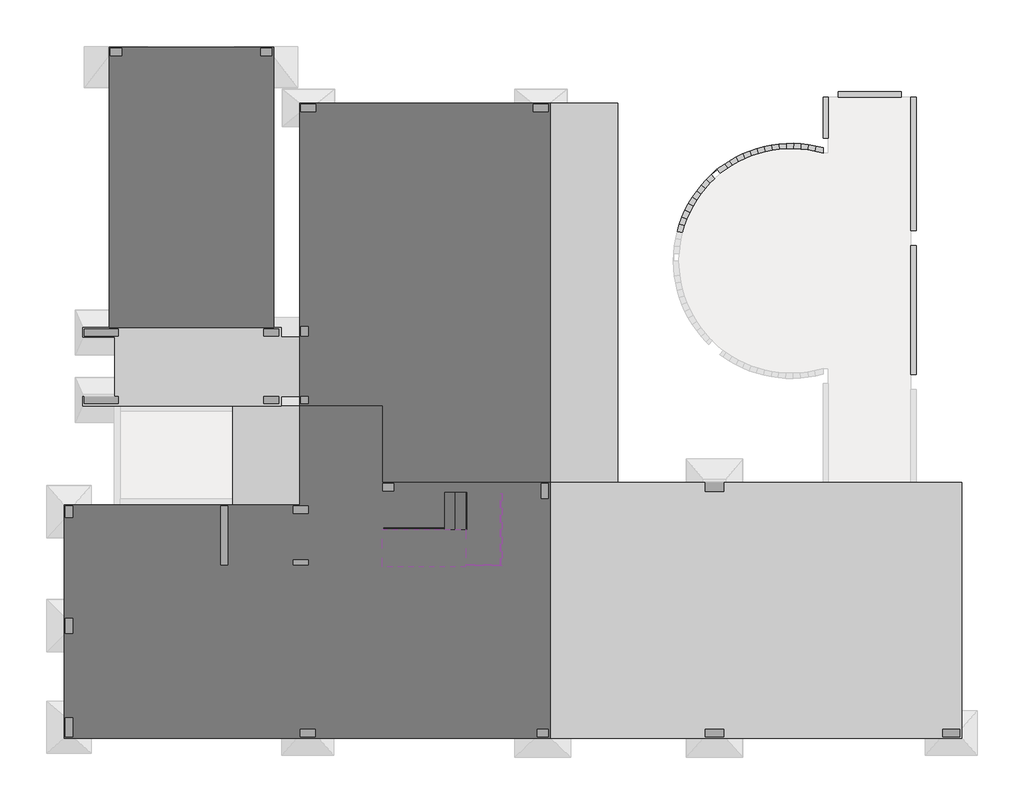
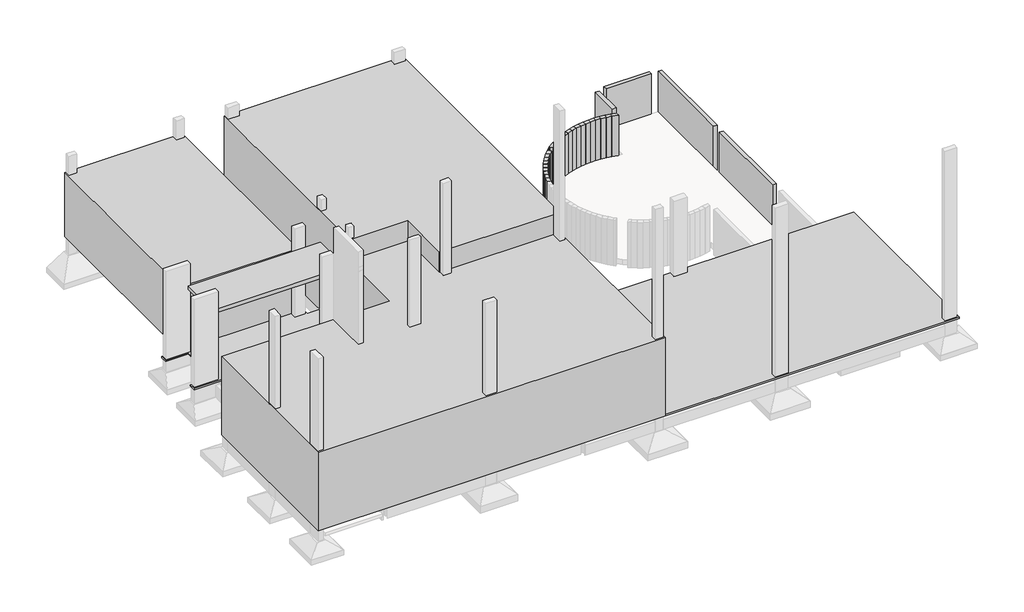
# One storey, part 4 of 4: 27 beams, 7 proxies, 6 railings, 2 stair flights, 1 slab.
# Revit data of these elements (continued)
# Element 2 (IfcBeam, "TQS - Viga retangular : 14.0 x 180.0") (continued)
#   Titulo = "VP6"
#   Chave = "-1017"
#   Tipo Elemento = "Viga"
#   SHA1 = "22C0BDACD46D49F6E4190D80621E2138C68CD36C"
#   Revisão = ""
#   Tipo de carga = ""
#   Divisor de flexao = ""
#   Secao = ""
#   Configuracao = ""
#   Angulo (graus) = ""
#   Detalhamento = ""
#   Casos de vento manual = ""
#   Tipo = ""
#   Alcas = ""
#   Furos = ""
#   Pino = ""
#   Distribuicao = ""
#   Solidarizado = ""
#   Solidarizar na montagem = ""
#   Unir com o próximo = ""
#   Grupo pre moldado = ""
#   Verificado = ""
#   Concreto C = ""
#   Taxa de armadura (kgf/m³) = 0
#   Carga (tf/m²) = 0
#   Carga (tf/m) = 0
#   Carga (tf) = 0
#   Altura = 1.80 m
#   Rebaixo = 0.15 m
#   Largura = 0.14 m
#   Distancia a face = 0.00 m
#   Distancia ao eixo = 0.00 m
#   Altura gerber esquerda = 0.00 m
#   Largura gerber esquerda = 0.00 m
#   Altura gerber direita = 0.00 m
#   Largura gerber direita = 0.00 m
#   Resultado de Ensaios fck (MPa) = 0
#   Unique TQS ID = -1017
#   Principal = yes
#   Structural Material = none
#   Phase Created = CC_AP/ESTR
# Element 3 (IfcBeam, "TQS - Viga retangular : 14.0 x 180.0")
#   Uso = "ESTRUTURA"
#   Titulo = "VP6"
#   Chave = "-1018"
#   Tipo Elemento = "Viga"
#   SHA1 = "D04A2C827C3C8BC1853343DA7F217DB9B9B2F05D"
#   Revisão = ""
#   Tipo de carga = ""
#   Divisor de flexao = ""
#   Secao = ""
#   Configuracao = ""
#   Angulo (graus) = ""
#   Detalhamento = ""
#   Casos de vento manual = ""
#   Tipo = ""
#   Alcas = ""
#   Furos = ""
#   Pino = ""
#   Distribuicao = ""
#   Solidarizado = ""
#   Solidarizar na montagem = ""
#   Unir com o próximo = ""
#   Grupo pre moldado = ""
#   Verificado = ""
#   Concreto C = ""
#   Taxa de armadura (kgf/m³) = 0
#   Carga (tf/m²) = 0
#   Carga (tf/m) = 0
#   Carga (tf) = 0
#   Altura = 1.80 m
#   Rebaixo = 0.15 m
#   Largura = 0.14 m
#   Distancia a face = 0.00 m
#   Distancia ao eixo = 0.00 m
#   Altura gerber esquerda = 0.00 m
#   Largura gerber esquerda = 0.00 m
#   Altura gerber direita = 0.00 m
#   Largura gerber direita = 0.00 m
#   Resultado de Ensaios fck (MPa) = 0
#   Unique TQS ID = -1018
#   Principal = yes
#   Structural Material = none
#   Phase Created = CC_AP/ESTR
# Element 4 (IfcBeam, "TQS - Viga retangular : 14.0 x 180.0")
#   Uso = "ESTRUTURA"
#   Titulo = "VP6"
#   Chave = "-1019"
#   Tipo Elemento = "Viga"
#   SHA1 = "0D182E2612785E293A5A4969EBA47990CD3E9117"
#   Revisão = ""
#   Tipo de carga = ""
#   Divisor de flexao = ""
#   Secao = ""
#   Configuracao = ""
#   Angulo (graus) = ""
#   Detalhamento = ""
#   Casos de vento manual = ""
#   Tipo = ""
#   Alcas = ""
#   Furos = ""
#   Pino = ""
#   Distribuicao = ""
#   Solidarizado = ""
#   Solidarizar na montagem = ""
#   Unir com o próximo = ""
#   Grupo pre moldado = ""
#   Verificado = ""
#   Concreto C = ""
#   Taxa de armadura (kgf/m³) = 0
#   Carga (tf/m²) = 0
#   Carga (tf/m) = 0
#   Carga (tf) = 0
#   Altura = 1.80 m
#   Rebaixo = 0.15 m
#   Largura = 0.14 m
#   Distancia a face = 0.00 m
#   Distancia ao eixo = 0.00 m
#   Altura gerber esquerda = 0.00 m
#   Largura gerber esquerda = 0.00 m
#   Altura gerber direita = 0.00 m
#   Largura gerber direita = 0.00 m
#   Resultado de Ensaios fck (MPa) = 0
#   Unique TQS ID = -1019
#   Principal = yes
#   Structural Material = none
#   Phase Created = CC_AP/ESTR
# Element 5 (IfcBeam, "TQS - Viga retangular : 14.0 x 180.0")
#   Uso = "ESTRUTURA"
#   Titulo = "VP6"
#   Chave = "-1020"
#   Tipo Elemento = "Viga"
#   SHA1 = "8A5DF36B72EBE22F2A453D6F9BADDE3EA3E2A9B4"
#   Revisão = ""
#   Tipo de carga = ""
#   Divisor de flexao = ""
#   Secao = ""
#   Configuracao = ""
#   Angulo (graus) = ""
#   Detalhamento = ""
#   Casos de vento manual = ""
#   Tipo = ""
#   Alcas = ""
#   Furos = ""
#   Pino = ""
#   Distribuicao = ""
#   Solidarizado = ""
#   Solidarizar na montagem = ""
#   Unir com o próximo = ""
#   Grupo pre moldado = ""
#   Verificado = ""
#   Concreto C = ""
#   Taxa de armadura (kgf/m³) = 0
#   Carga (tf/m²) = 0
#   Carga (tf/m) = 0
#   Carga (tf) = 0
#   Altura = 1.80 m
#   Rebaixo = 0.15 m
#   Largura = 0.14 m
#   Distancia a face = 0.00 m
#   Distancia ao eixo = 0.00 m
#   Altura gerber esquerda = 0.00 m
#   Largura gerber esquerda = 0.00 m
#   Altura gerber direita = 0.00 m
#   Largura gerber direita = 0.00 m
#   Resultado de Ensaios fck (MPa) = 0
#   Unique TQS ID = -1020
#   Principal = yes
#   Structural Material = none
#   Phase Created = CC_AP/ESTR
# Element 6 (IfcBeam, "TQS - Viga retangular : 14.0 x 180.0")
#   Uso = "ESTRUTURA"
#   Titulo = "VP6"
#   Chave = "-1021"
#   Tipo Elemento = "Viga"
#   SHA1 = "E996D88AC41B572457E87FBE2BFAA83C91B590B4"
#   Revisão = ""
#   Tipo de carga = ""
#   Divisor de flexao = ""
#   Secao = ""
#   Configuracao = ""
#   Angulo (graus) = ""
#   Detalhamento = ""
#   Casos de vento manual = ""
#   Tipo = ""
#   Alcas = ""
#   Furos = ""
#   Pino = ""
#   Distribuicao = ""
#   Solidarizado = ""
#   Solidarizar na montagem = ""
#   Unir com o próximo = ""
#   Grupo pre moldado = ""
#   Verificado = ""
#   Concreto C = ""
#   Taxa de armadura (kgf/m³) = 0
#   Carga (tf/m²) = 0
#   Carga (tf/m) = 0
#   Carga (tf) = 0
#   Altura = 1.80 m
#   Rebaixo = 0.15 m
#   Largura = 0.14 m
#   Distancia a face = 0.00 m
#   Distancia ao eixo = 0.00 m
#   Altura gerber esquerda = 0.00 m
#   Largura gerber esquerda = 0.00 m
#   Altura gerber direita = 0.00 m
#   Largura gerber direita = 0.00 m
#   Resultado de Ensaios fck (MPa) = 0
#   Unique TQS ID = -1021
#   Principal = yes
#   Structural Material = none
#   Phase Created = CC_AP/ESTR
# Element 7 (IfcBeam, "TQS - Viga retangular : 14.0 x 180.0")
#   Uso = "ESTRUTURA"
#   Titulo = "VP6"
#   Chave = "-1022"
#   Tipo Elemento = "Viga"
#   SHA1 = "0B33ED0C5CE953F65B7DD0F51C60662F46F82846"
#   Revisão = ""
#   Tipo de carga = ""
#   Divisor de flexao = ""
#   Secao = ""
#   Configuracao = ""
#   Angulo (graus) = ""
#   Detalhamento = ""
#   Casos de vento manual = ""
#   Tipo = ""
#   Alcas = ""
#   Furos = ""
#   Pino = ""
#   Distribuicao = ""
#   Solidarizado = ""
#   Solidarizar na montagem = ""
#   Unir com o próximo = ""
#   Grupo pre moldado = ""
#   Verificado = ""
#   Concreto C = ""
#   Taxa de armadura (kgf/m³) = 0
#   Carga (tf/m²) = 0
#   Carga (tf/m) = 0
#   Carga (tf) = 0
#   Altura = 1.80 m
#   Rebaixo = 0.15 m
#   Largura = 0.14 m
#   Distancia a face = 0.00 m
#   Distancia ao eixo = 0.00 m
#   Altura gerber esquerda = 0.00 m
#   Largura gerber esquerda = 0.00 m
#   Altura gerber direita = 0.00 m
#   Largura gerber direita = 0.00 m
#   Resultado de Ensaios fck (MPa) = 0
#   Unique TQS ID = -1022
#   Principal = yes
#   Structural Material = none
#   Phase Created = CC_AP/ESTR
# Element 8 (IfcBeam, "TQS - Viga retangular : 14.0 x 180.0")
#   Uso = "ESTRUTURA"
#   Titulo = "VP6"
#   Chave = "-1023"
#   Tipo Elemento = "Viga"
#   SHA1 = "7A0208B774D9472BDEB9F4D9C600465610707295"
#   Revisão = ""
#   Tipo de carga = ""
#   Divisor de flexao = ""
#   Secao = ""
#   Configuracao = ""
#   Angulo (graus) = ""
#   Detalhamento = ""
#   Casos de vento manual = ""
#   Tipo = ""
#   Alcas = ""
#   Furos = ""
#   Pino = ""
#   Distribuicao = ""
#   Solidarizado = ""
#   Solidarizar na montagem = ""
#   Unir com o próximo = ""
#   Grupo pre moldado = ""
#   Verificado = ""
#   Concreto C = ""
#   Taxa de armadura (kgf/m³) = 0
#   Carga (tf/m²) = 0
#   Carga (tf/m) = 0
#   Carga (tf) = 0
#   Altura = 1.80 m
#   Rebaixo = 0.15 m
#   Largura = 0.14 m
#   Distancia a face = 0.00 m
#   Distancia ao eixo = 0.00 m
#   Altura gerber esquerda = 0.00 m
#   Largura gerber esquerda = 0.00 m
#   Altura gerber direita = 0.00 m
#   Largura gerber direita = 0.00 m
#   Resultado de Ensaios fck (MPa) = 0
#   Unique TQS ID = -1023
#   Principal = yes
#   Structural Material = none
#   Phase Created = CC_AP/ESTR
# Element 9 (IfcBeam, "TQS - Viga retangular : 14.0 x 180.0")
#   Uso = "ESTRUTURA"
#   Titulo = "VP6"
#   Chave = "-1024"
#   Tipo Elemento = "Viga"
#   SHA1 = "84182F31E964F02A91D7472A67EEC15D959BEA6F"
#   Revisão = ""
#   Tipo de carga = ""
#   Divisor de flexao = ""
#   Secao = ""
#   Configuracao = ""
#   Angulo (graus) = ""
#   Detalhamento = ""
#   Casos de vento manual = ""
#   Tipo = ""
#   Alcas = ""
#   Furos = ""
#   Pino = ""
#   Distribuicao = ""
#   Solidarizado = ""
#   Solidarizar na montagem = ""
#   Unir com o próximo = ""
#   Grupo pre moldado = ""
#   Verificado = ""
#   Concreto C = ""
#   Taxa de armadura (kgf/m³) = 0
#   Carga (tf/m²) = 0
#   Carga (tf/m) = 0
#   Carga (tf) = 0
#   Altura = 1.80 m
#   Rebaixo = 0.15 m
#   Largura = 0.14 m
#   Distancia a face = 0.00 m
#   Distancia ao eixo = 0.00 m
#   Altura gerber esquerda = 0.00 m
#   Largura gerber esquerda = 0.00 m
#   Altura gerber direita = 0.00 m
#   Largura gerber direita = 0.00 m
#   Resultado de Ensaios fck (MPa) = 0
#   Unique TQS ID = -1024
#   Principal = yes
#   Structural Material = none
#   Phase Created = CC_AP/ESTR
# Element 10 (IfcBeam, "TQS - Viga retangular : 14.0 x 180.0")
#   Uso = "ESTRUTURA"
#   Titulo = "VP6"
#   Chave = "-1025"
#   Tipo Elemento = "Viga"
#   SHA1 = "018AD11D8442C61DF0F4C6D5519537CB9DF1785E"
#   Revisão = ""
#   Tipo de carga = ""
#   Divisor de flexao = ""
#   Secao = ""
#   Configuracao = ""
#   Angulo (graus) = ""
#   Detalhamento = ""
#   Casos de vento manual = ""
#   Tipo = ""
#   Alcas = ""
#   Furos = ""
#   Pino = ""
#   Distribuicao = ""
#   Solidarizado = ""
#   Solidarizar na montagem = ""
#   Unir com o próximo = ""
#   Grupo pre moldado = ""
#   Verificado = ""
#   Concreto C = ""
#   Taxa de armadura (kgf/m³) = 0
#   Carga (tf/m²) = 0
#   Carga (tf/m) = 0
#   Carga (tf) = 0
#   Altura = 1.80 m
#   Rebaixo = 0.15 m
#   Largura = 0.14 m
#   Distancia a face = 0.00 m
#   Distancia ao eixo = 0.00 m
#   Altura gerber esquerda = 0.00 m
#   Largura gerber esquerda = 0.00 m
#   Altura gerber direita = 0.00 m
#   Largura gerber direita = 0.00 m
#   Resultado de Ensaios fck (MPa) = 0
#   Unique TQS ID = -1025
#   Principal = yes
#   Structural Material = none
#   Phase Created = CC_AP/ESTR
# Element 11 (IfcBeam, "TQS - Viga retangular : 14.0 x 180.0")
#   Uso = "ESTRUTURA"
#   Titulo = "VP7"
#   Chave = "-1026"
#   Tipo Elemento = "Viga"
#   SHA1 = "EE0903180FC4F74752EE8D351596400DB6C4E3D3"
#   Revisão = ""
#   Tipo de carga = ""
#   Divisor de flexao = ""
#   Secao = ""
#   Configuracao = ""
#   Angulo (graus) = ""
#   Detalhamento = ""
#   Casos de vento manual = ""
#   Tipo = ""
#   Alcas = ""
#   Furos = ""
#   Pino = ""
#   Distribuicao = ""
#   Solidarizado = ""
#   Solidarizar na montagem = ""
#   Unir com o próximo = ""
#   Grupo pre moldado = ""
#   Verificado = ""
#   Concreto C = ""
#   Taxa de armadura (kgf/m³) = 0
#   Carga (tf/m²) = 0
#   Carga (tf/m) = 0
#   Carga (tf) = 0
#   Altura = 1.80 m
#   Rebaixo = 0.15 m
#   Largura = 0.14 m
#   Distancia a face = 0.00 m
#   Distancia ao eixo = 0.00 m
#   Altura gerber esquerda = 0.00 m
#   Largura gerber esquerda = 0.00 m
#   Altura gerber direita = 0.00 m
#   Largura gerber direita = 0.00 m
#   Resultado de Ensaios fck (MPa) = 0
#   Unique TQS ID = -1026
#   Principal = yes
#   Structural Material = none
#   Phase Created = CC_AP/ESTR
# Element 12 (IfcBeam, "TQS - Viga retangular : 14.0 x 180.0")
#   Uso = "ESTRUTURA"
#   Titulo = "VP7"
#   Chave = "-1027"
#   Tipo Elemento = "Viga"
#   SHA1 = "9C0E264E63AB224DB050780EBEBCCF0090D66D0A"
#   Revisão = ""
#   Tipo de carga = ""
#   Divisor de flexao = ""
#   Secao = ""
#   Configuracao = ""
#   Angulo (graus) = ""
#   Detalhamento = ""
#   Casos de vento manual = ""
#   Tipo = ""
#   Alcas = ""
#   Furos = ""
#   Pino = ""
#   Distribuicao = ""
#   Solidarizado = ""
#   Solidarizar na montagem = ""
#   Unir com o próximo = ""
#   Grupo pre moldado = ""
#   Verificado = ""
#   Concreto C = ""
#   Taxa de armadura (kgf/m³) = 0
#   Carga (tf/m²) = 0
#   Carga (tf/m) = 0
#   Carga (tf) = 0
#   Altura = 1.80 m
#   Rebaixo = 0.15 m
#   Largura = 0.14 m
#   Distancia a face = 0.00 m
#   Distancia ao eixo = 0.00 m
#   Altura gerber esquerda = 0.00 m
#   Largura gerber esquerda = 0.00 m
#   Altura gerber direita = 0.00 m
#   Largura gerber direita = 0.00 m
#   Resultado de Ensaios fck (MPa) = 0
#   Unique TQS ID = -1027
#   Principal = yes
#   Structural Material = none
#   Phase Created = CC_AP/ESTR
# Element 13 (IfcBeam, "TQS - Viga retangular : 14.0 x 180.0")
#   Uso = "ESTRUTURA"
#   Titulo = "VP7"
#   Chave = "-1028"
#   Tipo Elemento = "Viga"
#   SHA1 = "6E997BB4E590CA8C89FDA8B6D3FF6154DFE7002F"
#   Revisão = ""
#   Tipo de carga = ""
#   Divisor de flexao = ""
#   Secao = ""
#   Configuracao = ""
#   Angulo (graus) = ""
#   Detalhamento = ""
#   Casos de vento manual = ""
#   Tipo = ""
#   Alcas = ""
#   Furos = ""
#   Pino = ""
#   Distribuicao = ""
#   Solidarizado = ""
#   Solidarizar na montagem = ""
#   Unir com o próximo = ""
#   Grupo pre moldado = ""
#   Verificado = ""
#   Concreto C = ""
#   Taxa de armadura (kgf/m³) = 0
#   Carga (tf/m²) = 0
#   Carga (tf/m) = 0
#   Carga (tf) = 0
#   Altura = 1.80 m
#   Rebaixo = 0.15 m
#   Largura = 0.14 m
#   Distancia a face = 0.00 m
#   Distancia ao eixo = 0.00 m
#   Altura gerber esquerda = 0.00 m
#   Largura gerber esquerda = 0.00 m
#   Altura gerber direita = 0.00 m
#   Largura gerber direita = 0.00 m
#   Resultado de Ensaios fck (MPa) = 0
#   Unique TQS ID = -1028
#   Principal = yes
#   Structural Material = none
#   Phase Created = CC_AP/ESTR
# Element 14 (IfcBeam, "TQS - Viga retangular : 14.0 x 180.0")
#   Uso = "ESTRUTURA"
#   Titulo = "VP7"
#   Chave = "-1029"
#   Tipo Elemento = "Viga"
#   SHA1 = "7DDF74561A6D880C43286526A234CDA9ECB81B66"
#   Revisão = ""
#   Tipo de carga = ""
#   Divisor de flexao = ""
#   Secao = ""
#   Configuracao = ""
#   Angulo (graus) = ""
#   Detalhamento = ""
#   Casos de vento manual = ""
#   Tipo = ""
#   Alcas = ""
#   Furos = ""
#   Pino = ""
#   Distribuicao = ""
#   Solidarizado = ""
#   Solidarizar na montagem = ""
#   Unir com o próximo = ""
#   Grupo pre moldado = ""
#   Verificado = ""
#   Concreto C = ""
#   Taxa de armadura (kgf/m³) = 0
#   Carga (tf/m²) = 0
#   Carga (tf/m) = 0
#   Carga (tf) = 0
#   Altura = 1.80 m
#   Rebaixo = 0.15 m
#   Largura = 0.14 m
#   Distancia a face = 0.00 m
#   Distancia ao eixo = 0.00 m
#   Altura gerber esquerda = 0.00 m
#   Largura gerber esquerda = 0.00 m
#   Altura gerber direita = 0.00 m
#   Largura gerber direita = 0.00 m
#   Resultado de Ensaios fck (MPa) = 0
#   Unique TQS ID = -1029
#   Principal = yes
#   Structural Material = none
#   Phase Created = CC_AP/ESTR
# Element 15 (IfcBeam, "TQS - Viga retangular : 14.0 x 180.0")
#   Uso = "ESTRUTURA"
#   Titulo = "VP7"
#   Chave = "-1030"
#   Tipo Elemento = "Viga"
#   SHA1 = "2D411C14CB7CE55D4F1E0A23351751B1C30F9CC4"
#   Revisão = ""
#   Tipo de carga = ""
#   Divisor de flexao = ""
#   Secao = ""
#   Configuracao = ""
#   Angulo (graus) = ""
#   Detalhamento = ""
#   Casos de vento manual = ""
#   Tipo = ""
#   Alcas = ""
#   Furos = ""
#   Pino = ""
#   Distribuicao = ""
#   Solidarizado = ""
#   Solidarizar na montagem = ""
#   Unir com o próximo = ""
#   Grupo pre moldado = ""
#   Verificado = ""
#   Concreto C = ""
#   Taxa de armadura (kgf/m³) = 0
#   Carga (tf/m²) = 0
#   Carga (tf/m) = 0
#   Carga (tf) = 0
#   Altura = 1.80 m
#   Rebaixo = 0.15 m
#   Largura = 0.14 m
#   Distancia a face = 0.00 m
#   Distancia ao eixo = 0.00 m
#   Altura gerber esquerda = 0.00 m
#   Largura gerber esquerda = 0.00 m
#   Altura gerber direita = 0.00 m
#   Largura gerber direita = 0.00 m
#   Resultado de Ensaios fck (MPa) = 0
#   Unique TQS ID = -1030
#   Principal = yes
#   Structural Material = none
#   Phase Created = CC_AP/ESTR
# Element 16 (IfcBeam, "TQS - Viga retangular : 14.0 x 180.0")
#   Uso = "ESTRUTURA"
#   Titulo = "VP7"
#   Chave = "-1031"
#   Tipo Elemento = "Viga"
#   SHA1 = "171049F04C5F75504E61353FF9C8DE909D3AD5A1"
#   Revisão = ""
#   Tipo de carga = ""
#   Divisor de flexao = ""
#   Secao = ""
#   Configuracao = ""
#   Angulo (graus) = ""
#   Detalhamento = ""
#   Casos de vento manual = ""
#   Tipo = ""
#   Alcas = ""
#   Furos = ""
#   Pino = ""
#   Distribuicao = ""
#   Solidarizado = ""
#   Solidarizar na montagem = ""
#   Unir com o próximo = ""
#   Grupo pre moldado = ""
#   Verificado = ""
#   Concreto C = ""
#   Taxa de armadura (kgf/m³) = 0
#   Carga (tf/m²) = 0
#   Carga (tf/m) = 0
#   Carga (tf) = 0
#   Altura = 1.80 m
#   Rebaixo = 0.15 m
#   Largura = 0.14 m
#   Distancia a face = 0.00 m
#   Distancia ao eixo = 0.00 m
#   Altura gerber esquerda = 0.00 m
#   Largura gerber esquerda = 0.00 m
#   Altura gerber direita = 0.00 m
#   Largura gerber direita = 0.00 m
#   Resultado de Ensaios fck (MPa) = 0
#   Unique TQS ID = -1031
#   Principal = yes
#   Structural Material = none
#   Phase Created = CC_AP/ESTR
# Element 17 (IfcBeam, "TQS - Viga retangular : 14.0 x 180.0")
#   Uso = "ESTRUTURA"
#   Titulo = "VP7"
#   Chave = "-1032"
#   Tipo Elemento = "Viga"
#   SHA1 = "6DF824D13F17D5A6128940B40DFD1C2714CD6B1E"
#   Revisão = ""
#   Tipo de carga = ""
#   Divisor de flexao = ""
#   Secao = ""
#   Configuracao = ""
#   Angulo (graus) = ""
#   Detalhamento = ""
#   Casos de vento manual = ""
#   Tipo = ""
#   Alcas = ""
#   Furos = ""
#   Pino = ""
#   Distribuicao = ""
#   Solidarizado = ""
#   Solidarizar na montagem = ""
#   Unir com o próximo = ""
#   Grupo pre moldado = ""
#   Verificado = ""
#   Concreto C = ""
#   Taxa de armadura (kgf/m³) = 0
#   Carga (tf/m²) = 0
#   Carga (tf/m) = 0
#   Carga (tf) = 0
#   Altura = 1.80 m
#   Rebaixo = 0.15 m
#   Largura = 0.14 m
#   Distancia a face = 0.00 m
#   Distancia ao eixo = 0.00 m
#   Altura gerber esquerda = 0.00 m
#   Largura gerber esquerda = 0.00 m
#   Altura gerber direita = 0.00 m
#   Largura gerber direita = 0.00 m
#   Resultado de Ensaios fck (MPa) = 0
#   Unique TQS ID = -1032
#   Principal = yes
#   Structural Material = none
#   Phase Created = CC_AP/ESTR
# Element 18 (IfcBeam, "TQS - Viga retangular : 14.0 x 180.0")
#   Uso = "ESTRUTURA"
#   Titulo = "VP7"
#   Chave = "-1033"
#   Tipo Elemento = "Viga"
#   SHA1 = "2A35CBBA7314E7981D7057AA3DC248078908D855"
#   Revisão = ""
#   Tipo de carga = ""
#   Divisor de flexao = ""
#   Secao = ""
#   Configuracao = ""
#   Angulo (graus) = ""
#   Detalhamento = ""
#   Casos de vento manual = ""
#   Tipo = ""
#   Alcas = ""
#   Furos = ""
#   Pino = ""
#   Distribuicao = ""
#   Solidarizado = ""
#   Solidarizar na montagem = ""
#   Unir com o próximo = ""
#   Grupo pre moldado = ""
#   Verificado = ""
#   Concreto C = ""
#   Taxa de armadura (kgf/m³) = 0
#   Carga (tf/m²) = 0
#   Carga (tf/m) = 0
#   Carga (tf) = 0
#   Altura = 1.80 m
#   Rebaixo = 0.15 m
#   Largura = 0.14 m
#   Distancia a face = 0.00 m
#   Distancia ao eixo = 0.00 m
#   Altura gerber esquerda = 0.00 m
#   Largura gerber esquerda = 0.00 m
#   Altura gerber direita = 0.00 m
#   Largura gerber direita = 0.00 m
#   Resultado de Ensaios fck (MPa) = 0
#   Unique TQS ID = -1033
#   Principal = yes
#   Structural Material = none
#   Phase Created = CC_AP/ESTR
# Element 19 (IfcBeam, "TQS - Viga retangular : 14.0 x 180.0")
#   Uso = "ESTRUTURA"
#   Titulo = "VP7"
#   Chave = "-1034"
#   Tipo Elemento = "Viga"
#   SHA1 = "2B52F4D055F474E9CD7666D6686E78183A6E7EC4"
#   Revisão = ""
#   Tipo de carga = ""
#   Divisor de flexao = ""
#   Secao = ""
#   Configuracao = ""
#   Angulo (graus) = ""
#   Detalhamento = ""
#   Casos de vento manual = ""
#   Tipo = ""
#   Alcas = ""
#   Furos = ""
#   Pino = ""
#   Distribuicao = ""
#   Solidarizado = ""
#   Solidarizar na montagem = ""
#   Unir com o próximo = ""
#   Grupo pre moldado = ""
#   Verificado = ""
#   Concreto C = ""
#   Taxa de armadura (kgf/m³) = 0
#   Carga (tf/m²) = 0
#   Carga (tf/m) = 0
#   Carga (tf) = 0
#   Altura = 1.80 m
#   Rebaixo = 0.15 m
#   Largura = 0.14 m
#   Distancia a face = 0.00 m
#   Distancia ao eixo = 0.00 m
#   Altura gerber esquerda = 0.00 m
#   Largura gerber esquerda = 0.00 m
#   Altura gerber direita = 0.00 m
#   Largura gerber direita = 0.00 m
#   Resultado de Ensaios fck (MPa) = 0
#   Unique TQS ID = -1034
#   Principal = yes
#   Structural Material = none
#   Phase Created = CC_AP/ESTR
# Element 20 (IfcBeam, "TQS - Viga retangular : 14.0 x 180.0")
#   Uso = "ESTRUTURA"
#   Titulo = "VP7"
#   Chave = "-1035"
#   Tipo Elemento = "Viga"
#   SHA1 = "4164F1A2AAB45DB19362C3FEFBBEE02BFBC2F3D5"
#   Revisão = ""
#   Tipo de carga = ""
#   Divisor de flexao = ""
#   Secao = ""
#   Configuracao = ""
#   Angulo (graus) = ""
#   Detalhamento = ""
#   Casos de vento manual = ""
#   Tipo = ""
#   Alcas = ""
#   Furos = ""
#   Pino = ""
#   Distribuicao = ""
#   Solidarizado = ""
#   Solidarizar na montagem = ""
#   Unir com o próximo = ""
#   Grupo pre moldado = ""
#   Verificado = ""
#   Concreto C = ""
#   Taxa de armadura (kgf/m³) = 0
#   Carga (tf/m²) = 0
#   Carga (tf/m) = 0
#   Carga (tf) = 0
#   Altura = 1.80 m
#   Rebaixo = 0.15 m
#   Largura = 0.14 m
#   Distancia a face = 0.00 m
#   Distancia ao eixo = 0.00 m
#   Altura gerber esquerda = 0.00 m
#   Largura gerber esquerda = 0.00 m
#   Altura gerber direita = 0.00 m
#   Largura gerber direita = 0.00 m
#   Resultado de Ensaios fck (MPa) = 0
#   Unique TQS ID = -1035
#   Principal = yes
#   Structural Material = none
#   Phase Created = CC_AP/ESTR
# Element 21 (IfcBeam, "TQS - Viga retangular : 14.0 x 180.0")
#   Uso = "ESTRUTURA"
#   Titulo = "VP7"
#   Chave = "-1036"
#   Tipo Elemento = "Viga"
#   SHA1 = "488CD87153485AFAB4498525AFF36ABFE92E7622"
#   Revisão = ""
#   Tipo de carga = ""
#   Divisor de flexao = ""
#   Secao = ""
#   Configuracao = ""
#   Angulo (graus) = ""
#   Detalhamento = ""
#   Casos de vento manual = ""
#   Tipo = ""
#   Alcas = ""
#   Furos = ""
#   Pino = ""
#   Distribuicao = ""
#   Solidarizado = ""
#   Solidarizar na montagem = ""
#   Unir com o próximo = ""
#   Grupo pre moldado = ""
#   Verificado = ""
#   Concreto C = ""
#   Taxa de armadura (kgf/m³) = 0
#   Carga (tf/m²) = 0
#   Carga (tf/m) = 0
#   Carga (tf) = 0
#   Altura = 1.80 m
#   Rebaixo = 0.15 m
#   Largura = 0.14 m
#   Distancia a face = 0.00 m
#   Distancia ao eixo = 0.00 m
#   Altura gerber esquerda = 0.00 m
#   Largura gerber esquerda = 0.00 m
#   Altura gerber direita = 0.00 m
#   Largura gerber direita = 0.00 m
#   Resultado de Ensaios fck (MPa) = 0
#   Unique TQS ID = -1036
#   Principal = yes
#   Structural Material = none
#   Phase Created = CC_AP/ESTR
# Element 22 (IfcBeam, "TQS - Viga retangular : 14.0 x 180.0")
#   Uso = "ESTRUTURA"
#   Titulo = "VP7"
#   Chave = "-1037"
#   Tipo Elemento = "Viga"
#   SHA1 = "197F68BC870D688E0A2EC9FD05BD8B81B3EE2891"
#   Revisão = ""
#   Tipo de carga = ""
#   Divisor de flexao = ""
#   Secao = ""
#   Configuracao = ""
#   Angulo (graus) = ""
#   Detalhamento = ""
#   Casos de vento manual = ""
#   Tipo = ""
#   Alcas = ""
#   Furos = ""
#   Pino = ""
#   Distribuicao = ""
#   Solidarizado = ""
#   Solidarizar na montagem = ""
#   Unir com o próximo = ""
#   Grupo pre moldado = ""
#   Verificado = ""
#   Concreto C = ""
#   Taxa de armadura (kgf/m³) = 0
#   Carga (tf/m²) = 0
#   Carga (tf/m) = 0
#   Carga (tf) = 0
#   Altura = 1.80 m
#   Rebaixo = 0.15 m
#   Largura = 0.14 m
#   Distancia a face = 0.00 m
#   Distancia ao eixo = 0.00 m
#   Altura gerber esquerda = 0.00 m
#   Largura gerber esquerda = 0.00 m
#   Altura gerber direita = 0.00 m
#   Largura gerber direita = 0.00 m
#   Resultado de Ensaios fck (MPa) = 0
#   Unique TQS ID = -1037
#   Principal = yes
#   Structural Material = none
#   Phase Created = CC_AP/ESTR
# Element 23 (IfcBeam, "TQS - Viga retangular : 14.0 x 180.0")
#   Uso = "ESTRUTURA"
#   Titulo = "VP7"
#   Chave = "-1038"
#   Tipo Elemento = "Viga"
#   SHA1 = "A01B41D9FF886BEAE3E617D97EE3619056D0B1F6"
#   Revisão = ""
#   Tipo de carga = ""
#   Divisor de flexao = ""
#   Secao = ""
#   Configuracao = ""
#   Angulo (graus) = ""
#   Detalhamento = ""
#   Casos de vento manual = ""
#   Tipo = ""
#   Alcas = ""
#   Furos = ""
#   Pino = ""
#   Distribuicao = ""
#   Solidarizado = ""
#   Solidarizar na montagem = ""
#   Unir com o próximo = ""
#   Grupo pre moldado = ""
#   Verificado = ""
#   Concreto C = ""
#   Taxa de armadura (kgf/m³) = 0
#   Carga (tf/m²) = 0
#   Carga (tf/m) = 0
#   Carga (tf) = 0
#   Altura = 1.80 m
#   Rebaixo = 0.15 m
#   Largura = 0.14 m
#   Distancia a face = 0.00 m
#   Distancia ao eixo = 0.00 m
#   Altura gerber esquerda = 0.00 m
#   Largura gerber esquerda = 0.00 m
#   Altura gerber direita = 0.00 m
#   Largura gerber direita = 0.00 m
#   Resultado de Ensaios fck (MPa) = 0
#   Unique TQS ID = -1038
#   Principal = yes
#   Structural Material = none
#   Phase Created = CC_AP/ESTR
# Element 24 (IfcBeam, "TQS - Viga retangular : 14.0 x 180.0")
#   Uso = "ESTRUTURA"
#   Titulo = "VP7"
#   Chave = "-1039"
#   Tipo Elemento = "Viga"
#   SHA1 = "464C06C93C140F0D2F14A56FBCB9B233FA9BCEFA"
#   Revisão = ""
#   Tipo de carga = ""
#   Divisor de flexao = ""
#   Secao = ""
#   Configuracao = ""
#   Angulo (graus) = ""
#   Detalhamento = ""
#   Casos de vento manual = ""
#   Tipo = ""
#   Alcas = ""
#   Furos = ""
#   Pino = ""
#   Distribuicao = ""
#   Solidarizado = ""
#   Solidarizar na montagem = ""
#   Unir com o próximo = ""
#   Grupo pre moldado = ""
#   Verificado = ""
#   Concreto C = ""
#   Taxa de armadura (kgf/m³) = 0
#   Carga (tf/m²) = 0
#   Carga (tf/m) = 0
#   Carga (tf) = 0
#   Altura = 1.80 m
#   Rebaixo = 0.15 m
#   Largura = 0.14 m
#   Distancia a face = 0.00 m
#   Distancia ao eixo = 0.00 m
#   Altura gerber esquerda = 0.00 m
#   Largura gerber esquerda = 0.00 m
#   Altura gerber direita = 0.00 m
#   Largura gerber direita = 0.00 m
#   Resultado de Ensaios fck (MPa) = 0
#   Unique TQS ID = -1039
#   Principal = yes
#   Structural Material = none
#   Phase Created = CC_AP/ESTR
# Element 25 (IfcBeam, "TQS - Viga retangular : 14.0 x 180.0")
#   Uso = "ESTRUTURA"
#   Titulo = "VP7"
#   Chave = "-1040"
#   Tipo Elemento = "Viga"
#   SHA1 = "4C21DE7F9DAC405A6DCBFB549F747162CD869074"
#   Revisão = ""
#   Tipo de carga = ""
#   Divisor de flexao = ""
#   Secao = ""
#   Configuracao = ""
#   Angulo (graus) = ""
#   Detalhamento = ""
#   Casos de vento manual = ""
#   Tipo = ""
#   Alcas = ""
#   Furos = ""
#   Pino = ""
#   Distribuicao = ""
#   Solidarizado = ""
#   Solidarizar na montagem = ""
#   Unir com o próximo = ""
#   Grupo pre moldado = ""
#   Verificado = ""
#   Concreto C = ""
#   Taxa de armadura (kgf/m³) = 0
#   Carga (tf/m²) = 0
#   Carga (tf/m) = 0
#   Carga (tf) = 0
#   Altura = 1.80 m
#   Rebaixo = 0.15 m
#   Largura = 0.14 m
#   Distancia a face = 0.00 m
#   Distancia ao eixo = 0.00 m
#   Altura gerber esquerda = 0.00 m
#   Largura gerber esquerda = 0.00 m
#   Altura gerber direita = 0.00 m
#   Largura gerber direita = 0.00 m
#   Resultado de Ensaios fck (MPa) = 0
#   Unique TQS ID = -1040
#   Principal = yes
#   Structural Material = none
#   Phase Created = CC_AP/ESTR
# Element 26 (IfcBeam, "TQS - Viga retangular : 14.0 x 180.0")
#   Uso = "ESTRUTURA"
#   Titulo = "VP8"
#   Chave = "-1041"
#   Tipo Elemento = "Viga"
#   SHA1 = "6AA3E4511FE5BFB69BE90AF5BC0D9228BA1EC532"
#   Revisão = ""
#   Tipo de carga = ""
#   Divisor de flexao = ""
#   Secao = ""
#   Configuracao = ""
#   Angulo (graus) = ""
#   Detalhamento = ""
#   Casos de vento manual = ""
#   Tipo = ""
#   Alcas = ""
#   Furos = ""
#   Pino = ""
#   Distribuicao = ""
#   Solidarizado = ""
#   Solidarizar na montagem = ""
#   Unir com o próximo = ""
#   Grupo pre moldado = ""
#   Verificado = ""
#   Concreto C = ""
#   Taxa de armadura (kgf/m³) = 0
#   Carga (tf/m²) = 0
#   Carga (tf/m) = 0
#   Carga (tf) = 0
#   Altura = 1.80 m
#   Rebaixo = 0.15 m
#   Largura = 0.14 m
#   Distancia a face = 0.00 m
#   Distancia ao eixo = 0.00 m
#   Altura gerber esquerda = 0.00 m
#   Largura gerber esquerda = 0.00 m
#   Altura gerber direita = 0.00 m
#   Largura gerber direita = 0.00 m
#   Resultado de Ensaios fck (MPa) = 0
#   Unique TQS ID = -1041
#   Principal = yes
#   Structural Material = none
#   Phase Created = CC_AP/ESTR
# Element 27 (IfcBeam, "TQS - Viga retangular : 14.0 x 180.0")
#   Uso = "ESTRUTURA"
#   Titulo = "VP10"
#   Chave = "-1044"
#   Tipo Elemento = "Viga"
#   SHA1 = "7E9D2D7EE297E45D169793BFEC03634A2C078807"
#   Revisão = ""
#   Tipo de carga = ""
#   Divisor de flexao = ""
#   Secao = ""
#   Configuracao = ""
#   Angulo (graus) = ""
#   Detalhamento = ""
#   Casos de vento manual = ""
#   Tipo = ""
#   Alcas = ""
#   Furos = ""
#   Pino = ""
#   Distribuicao = ""
#   Solidarizado = ""
#   Solidarizar na montagem = ""
#   Unir com o próximo = ""
#   Grupo pre moldado = ""
#   Verificado = ""
#   Concreto C = ""
#   Taxa de armadura (kgf/m³) = 0
#   Carga (tf/m²) = 0
#   Carga (tf/m) = 0
#   Carga (tf) = 0
#   Altura = 1.80 m
#   Rebaixo = 0.15 m
#   Largura = 0.14 m
#   Distancia a face = 0.00 m
#   Distancia ao eixo = 0.00 m
#   Altura gerber esquerda = 0.00 m
#   Largura gerber esquerda = 0.00 m
#   Altura gerber direita = 0.00 m
#   Largura gerber direita = 0.00 m
#   Resultado de Ensaios fck (MPa) = 0
#   Unique TQS ID = -1044
#   Principal = yes
#   Structural Material = none
#   Phase Created = CC_AP/ESTR
# Element 28 (IfcBuildingElementProxy, "GARAGEM : GARAGEM")
#   Phase Created = CC_EV
#   Materials on its faces: "Forma padrão"
# Element 29 (IfcBuildingElementProxy, "PERGOLADO SALAS : PERGOLADO SALAS")
#   Phase Created = CC_EV
#   Materials on its faces: "Forma padrão"
# Element 30 (IfcBuildingElementProxy, "VARANDA GOURMET : VARANDA GOURMET")
#   Phase Created = CC_EV
#   Materials on its faces: "Forma padrão"
# Element 31 (IfcBuildingElementProxy, "PÓRTICO ENTRADA : PÓRTICO ENTRADA")
#   Phase Created = CC_EV
#   Materials on its faces: "Forma padrão"
# Element 32 (IfcBuildingElementProxy, "SALAS : SALAS")
#   Phase Created = CC_EV
#   Materials on its faces: "Forma padrão"
# Element 33 (IfcBuildingElementProxy, "PROJEÇÃO : PROJEÇÃO")
#   Phase Created = CC_EV
#   Materials on its faces: "Forma padrão"
# Element 34 (IfcBuildingElementProxy, "COZINHA E LAVANDERIA : COZINHA E LAVANDERIA")
#   Phase Created = CC_EV
#   Materials on its faces: "Forma padrão"
# Element 35 (IfcRailing, "ML_Perfil U de embutir3 : ML_Perfil U de embutir")
#   Uso = "PATAMAR"
#   ME_Compr = 1.94 m
#   ME_Material Perfil = .ALUMÍNIO COM PINTURA ELETROSTÁTICA BRANCA
#   Phase Created = CC_AP
#   Materials on its faces: ".ALUMÍNIO COM PINTURA ELETROSTÁTICA BRANCA"
# Element 36 (IfcRailing, "ML_Painéis3 : ML_Painéis")
#   Uso = "PATAMAR"
#   ME_Área = 2.1296 m²
#   ME_Espessura = 0.012 m
#   ME_Dist Painéis = 0.002 m
#   ME_Compr Painéis = 1.936 m
#   ME_Compr = 1.94 m
#   ME_Altura = 1.10 m
#   ME_Quant Painéis = 3
#   ME_Painel Único = yes
#   ME_Paineis Vários = no
#   ME_Material Tipo Vidro = .VIDRO GENÉRICO
#   Phase Created = CC_AP
#   Materials on its faces: ".VIDRO GENÉRICO"
# Element 37 (IfcRailing, "ML_Perfil U de embutir4 : ML_Perfil U de embutir")
#   Uso = "PATAMAR"
#   ME_Compr = 0.925 m
#   ME_Material Perfil = .ALUMÍNIO COM PINTURA ELETROSTÁTICA BRANCA
#   Phase Created = CC_AP
#   Materials on its faces: ".ALUMÍNIO COM PINTURA ELETROSTÁTICA BRANCA"
# Element 38 (IfcRailing, "ML_Painéis4 : ML_Painéis")
#   Uso = "PATAMAR"
#   ME_Área = 1.0131 m²
#   ME_Espessura = 0.012 m
#   ME_Dist Painéis = 0.002 m
#   ME_Compr Painéis = 0.921 m
#   ME_Compr = 0.925 m
#   ME_Altura = 1.10 m
#   ME_Quant Painéis = 3
#   ME_Painel Único = yes
#   ME_Paineis Vários = no
#   ME_Material Tipo Vidro = .VIDRO GENÉRICO
#   Phase Created = CC_AP
#   Materials on its faces: ".VIDRO GENÉRICO"
# Element 39 (IfcRailing, "ML_Guarda_corpo lance : ML_Guarda_corpo lance")
#   Uso = "LANCE"
#   ME_Espessura = 0.012 m
#   ME_Material Tipo Vidro = .VIDRO GENÉRICO
#   Phase Created = CC_AP
#   Materials on its faces: ".VIDRO GENÉRICO"
# Element 40 (IfcRailing, "ML_Guarda_corpo lance1 : ML_Guarda_corpo lance")
#   Uso = "LANCE"
#   ME_Espessura = 0.012 m
#   ME_Material Tipo Vidro = .VIDRO GENÉRICO
#   Phase Created = CC_AP
#   Materials on its faces: ".VIDRO GENÉRICO"
# Element 41 (IfcSlab, "Espessura de 300 mm")
#   Phase Created = CC_AP
#   Materials on its faces: ".SOLEIRA DE CUMARÚ"
# Elements 42, 43 (IfcStairFlight, "Profundidade de 150 mm - SEM BOCEL")
#   Phase Created = CC_AP
#   Materials on its faces: ".SOLEIRA DE CUMARÚ", ".CONCRETO ESTRUTURAL"
# Materials
#   ".ALUMÍNIO COM PINTURA ELETROSTÁTICA BRANCA": class "CC_METAIS", colour RGB 241 241 241, transparency 0, Cost = 0
#   ".VIDRO GENÉRICO": class ".CC_VIDRO", colour RGB 0 128 192, transparency 0.9, Description = "Vidro comum", Cost = 0
#   "Forma padrão": class "Genérico", colour RGB 185 189 196, transparency 0.5, Cost = 0
#   ".SOLEIRA DE CUMARÚ": class ".CC_MADEIRAS", colour RGB 188 160 135, transparency 0, Cost = 0
#   ".CONCRETO ESTRUTURAL": class ".CC_CONCRETO", colour RGB 192 192 192, transparency 0, Description = "Concreto moldado no local", Cost = 0
